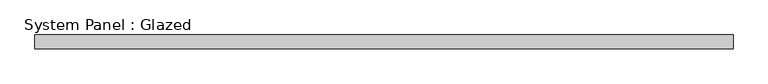
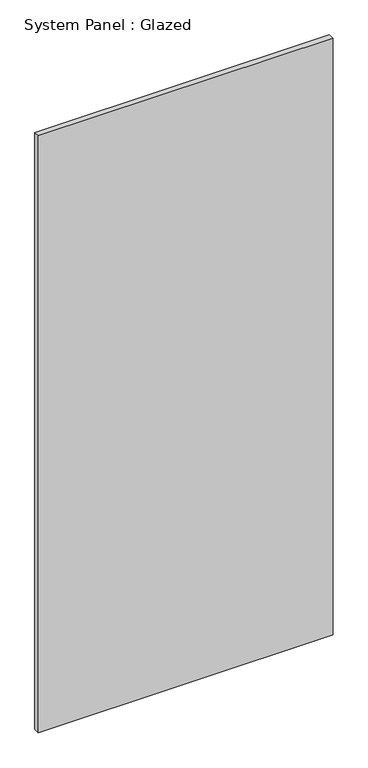
"""IFC4 building model written with IfcOpenShell, lengths in millimetres: plate geometry, System Panel : Glazed."""

import ifcopenshell
import ifcopenshell.guid

model = None  # the IFC model being written
_history = None  # IfcOwnerHistory: only IFC2X3 demands one
_inside = {}  # id of a spatial element -> (the spatial element, [elements in it])
_under = {}  # id of a project, library or spatial element -> (it, [spatial elements below it])
_declared = {}  # id of a project -> (the project, [libraries it declares])
_typed = {}  # id of a type object -> (the type object, [elements of that type])
_made_of = {}  # id of a material, layer set ... -> (it, [elements and type objects made of it])


def new_model(schema):
    """Start an empty IFC model of exactly this schema.

    Asked for "IFC4X3", IfcOpenShell would pick the latest addendum, in which some entities
    have other attributes; the version numbers below select the first issue.
    IFC2X3 requires an IfcOwnerHistory on every rooted entity: one is made here for all.
    """
    global model, _history
    if schema == "IFC4X3":
        model = ifcopenshell.file(schema_version=(4, 3, 0, 0))
    else:
        model = ifcopenshell.file(schema=schema)
    _inside.clear()
    _under.clear()
    _declared.clear()
    _typed.clear()
    _made_of.clear()
    _history = None
    if model.schema == "IFC2X3":
        org = make("IfcOrganization", Name="unknown")
        user = make(
            "IfcPersonAndOrganization",
            ThePerson=make("IfcPerson", FamilyName="unknown"),
            TheOrganization=org,
        )
        app = make(
            "IfcApplication",
            ApplicationDeveloper=org,
            Version="unknown",
            ApplicationFullName="unknown",
            ApplicationIdentifier="unknown",
        )
        _history = make(
            "IfcOwnerHistory",
            OwningUser=user,
            OwningApplication=app,
            ChangeAction="ADDED",
            CreationDate=0,
        )
    return model


def make(cls, **values):
    """One entity of the class cls with the attributes given. An attribute that is None is left unset."""
    return model.create_entity(
        cls, **{name: value for name, value in values.items() if value is not None}
    )


def rooted(cls, **values):
    """An entity with a GlobalId (a new one), such as an element, a storey or a relation."""
    return make(cls, GlobalId=ifcopenshell.guid.new(), OwnerHistory=_history, **values)


def si_unit(unit_type, name, prefix=None):
    """IfcSIUnit, for example si_unit("LENGTHUNIT", "METRE", prefix="MILLI")."""
    return make("IfcSIUnit", UnitType=unit_type, Prefix=prefix, Name=name)


def assignment(units):
    """IfcUnitAssignment: the units of a project."""
    return None if units is None else make("IfcUnitAssignment", Units=units)


def point(xyz):
    """IfcCartesianPoint."""
    return None if xyz is None else make("IfcCartesianPoint", Coordinates=xyz)


def direction(xyz):
    """IfcDirection."""
    return None if xyz is None else make("IfcDirection", DirectionRatios=xyz)


def frame(location, z_axis=None, x_axis=None):
    """IfcAxis2Placement3D, a coordinate frame: its origin and axes. An axis left out is left unset."""
    return make(
        "IfcAxis2Placement3D",
        Location=point(location),
        Axis=direction(z_axis),
        RefDirection=direction(x_axis),
    )


def origin():
    """The frame at (0, 0, 0) with its axes left unset."""
    return frame((0.0, 0.0, 0.0))


def origin_with_axes():
    """The frame at (0, 0, 0) with the z axis (0, 0, 1) and the x axis (1, 0, 0) written out."""
    return frame((0.0, 0.0, 0.0), z_axis=(0.0, 0.0, 1.0), x_axis=(1.0, 0.0, 0.0))


def place(relative_to, where):
    """IfcLocalPlacement: puts the frame where relative to a parent placement (None: the world)."""
    return make(
        "IfcLocalPlacement", PlacementRelTo=relative_to, RelativePlacement=where
    )


def context(
    kind, dimensions, precision=None, world=None, true_north=None, identifier=None
):
    """IfcGeometricRepresentationContext, for example the 3D "Model" context."""
    return make(
        "IfcGeometricRepresentationContext",
        ContextIdentifier=identifier,
        ContextType=kind,
        CoordinateSpaceDimension=dimensions,
        Precision=precision,
        WorldCoordinateSystem=world,
        TrueNorth=true_north,
    )


def project(units=None, contexts=None):
    """IfcProject with its units and contexts."""
    return rooted(
        "IfcProject",
        Name="project",
        RepresentationContexts=contexts,
        UnitsInContext=assignment(units),
    )


def spatial(cls, under=None, at=None, **own):
    """A site, building, storey or space (cls), placed at a placement, below another one or the project."""
    s = rooted(cls, ObjectPlacement=at, **own)
    if under is not None:
        _under.setdefault(under.id(), (under, []))[1].append(s)
    return s


def polyline(points):
    """IfcPolyline through the points."""
    return make("IfcPolyline", Points=[point(p) for p in points])


def outline(outer, holes=None, kind="AREA"):
    """IfcArbitraryClosedProfileDef: a profile drawn as a closed curve; with holes, ...WithVoids."""
    if holes is None:
        return make("IfcArbitraryClosedProfileDef", ProfileType=kind, OuterCurve=outer)
    return make(
        "IfcArbitraryProfileDefWithVoids",
        ProfileType=kind,
        OuterCurve=outer,
        InnerCurves=holes,
    )


def extrude(swept, where, along, depth):
    """IfcExtrudedAreaSolid: the profile swept, set in the frame where, extruded along a direction by depth."""
    return make(
        "IfcExtrudedAreaSolid",
        SweptArea=swept,
        Position=where,
        ExtrudedDirection=direction(along),
        Depth=depth,
    )


def shape(context_of_items, identifier, shape_type, items):
    """IfcShapeRepresentation: the items that make up one representation, for example the "Body"."""
    return make(
        "IfcShapeRepresentation",
        ContextOfItems=context_of_items,
        RepresentationIdentifier=identifier,
        RepresentationType=shape_type,
        Items=items,
    )


def source(mapping_origin, context_of_items, identifier, shape_type, items):
    """IfcRepresentationMap: a shape defined once, which mapped items show again and again."""
    return make(
        "IfcRepresentationMap",
        MappingOrigin=mapping_origin,
        MappedRepresentation=shape(context_of_items, identifier, shape_type, items),
    )


def transform(
    local_origin,
    x_axis=None,
    y_axis=None,
    z_axis=None,
    scale=None,
    scale2=None,
    scale3=None,
    uniform=True,
):
    """IfcCartesianTransformationOperator3D, or its non-uniform kind. x_axis, y_axis, z_axis: its Axis1, 2, 3."""
    if uniform:
        return make(
            "IfcCartesianTransformationOperator3D",
            Axis1=direction(x_axis),
            Axis2=direction(y_axis),
            LocalOrigin=point(local_origin),
            Scale=scale,
            Axis3=direction(z_axis),
        )
    return make(
        "IfcCartesianTransformationOperator3DnonUniform",
        Axis1=direction(x_axis),
        Axis2=direction(y_axis),
        LocalOrigin=point(local_origin),
        Scale=scale,
        Axis3=direction(z_axis),
        Scale2=scale2,
        Scale3=scale3,
    )


def mapped(mapping_source, mapping_target):
    """IfcMappedItem: shows the shape of a source again, moved by a transform."""
    return make(
        "IfcMappedItem", MappingSource=mapping_source, MappingTarget=mapping_target
    )


def made_of(thing, what):
    """Note that an element or type object is made of a material, layer set ...; save() writes the relation."""
    if what is not None:
        _made_of.setdefault(what.id(), (what, []))[1].append(thing)
    return thing


def element(
    cls,
    number,
    at=None,
    inside=None,
    cuts=None,
    type_object=None,
    material=None,
    context=None,
    identifier="Body",
    shape_type=None,
    held_by="IfcProductDefinitionShape",
    body=None,
    shapes=None,
    **own,
):
    """One element of the class cls, such as IfcWall. Its Tag is "e" and its number.

    at: its placement. inside: the storey or other place that contains it. cuts: it is an
    opening in that element (IfcRelVoidsElement). A single representation is given by context,
    identifier, shape_type and body (its items); several are given by shapes. held_by: the class
    of the entity that holds the representations. save() writes the other relations.
    """
    e = rooted(cls, Tag="e%d" % number, ObjectPlacement=at, **own)
    if body is not None:
        shapes = [shape(context, identifier, shape_type, body)]
    if shapes is not None:
        e.Representation = make(held_by, Representations=shapes)
    if inside is not None:
        _inside.setdefault(inside.id(), (inside, []))[1].append(e)
    if cuts is not None:
        rooted(
            "IfcRelVoidsElement", RelatingBuildingElement=cuts, RelatedOpeningElement=e
        )
    if type_object is not None:
        _typed.setdefault(type_object.id(), (type_object, []))[1].append(e)
    return made_of(e, material)


def aggregate(whole, parts):
    """IfcRelAggregates: a whole, such as a stair, and the parts it consists of."""
    return rooted("IfcRelAggregates", RelatingObject=whole, RelatedObjects=parts)


def save(model, path):
    """Write the relations noted so far, then the file.

    IfcRelAggregates (storeys below a building ...), IfcRelContainedInSpatialStructure (elements
    in a storey), IfcRelDefinesByType, IfcRelAssociatesMaterial and IfcRelDeclares: one each for
    every whole, place, type object, material and project.
    """
    for whole, parts in _under.values():
        aggregate(whole, parts)
    for where, things in _inside.values():
        rooted(
            "IfcRelContainedInSpatialStructure",
            RelatedElements=things,
            RelatingStructure=where,
        )
    for kind, things in _typed.values():
        rooted("IfcRelDefinesByType", RelatedObjects=things, RelatingType=kind)
    for what, things in _made_of.values():
        rooted("IfcRelAssociatesMaterial", RelatedObjects=things, RelatingMaterial=what)
    for by, libraries in _declared.values():
        rooted("IfcRelDeclares", RelatingContext=by, RelatedDefinitions=libraries)
    model.write(path)


def system_panel_glazed_36e52168(model_context):
    return source(origin(), model_context, "Body", "SweptSolid", [
        extrude(outline(polyline([(651.3841819, 19.05), (-651.3841819, 19.05), (-651.3841819, 44.45), (651.3841819, 44.45), (651.3841819, 19.05)])), origin_with_axes(), (0.0, 0.0, 1.0), 2788.92),
    ])


if __name__ == "__main__":
    model = new_model("IFC4")
    model_context = context("Model", 3, world=origin())
    ifc_project = project(units=[si_unit("LENGTHUNIT", "METRE", prefix="MILLI")], contexts=[model_context])
    site = spatial("IfcSite", under=ifc_project)
    building = spatial("IfcBuilding", under=site)
    placement = place(None, origin())
    system_panel_glazed_shape = system_panel_glazed_36e52168(model_context)
    element("IfcPlate", 1, ObjectType="System Panel : Glazed", at=placement, inside=building, context=model_context, shape_type="MappedRepresentation", body=[
        mapped(system_panel_glazed_shape, transform((0.0, 0.0, 0.0), x_axis=(1.0, 0.0, 0.0), y_axis=(0.0, 1.0, 0.0), z_axis=(0.0, 0.0, 1.0))),
    ])
    save(model, "model.ifc")

# Revit data of these elements
# Type "System Panel : Glazed"
#   Construction Type Id = "GSP4R"
#   Analytic Construction = "1/8 in Pilkington single glazing"
#   Visual Light Transmittance = 0.9
#   Solar Heat Gain Coefficient = 0.86
#   Heat Transfer Coefficient (U) = 1.18115 BTU/(h·ft²·°F)
#   Define Thermal Properties by = 1
# Element 1 (IfcPlate, "System Panel : Glazed")
#   Materials on its faces: "Glass"
# Materials
#   "Glass": class "Glass", colour RGB 0 128 192, transparency 0.75, Description = "Soda Lime Glass", Cost = 0
